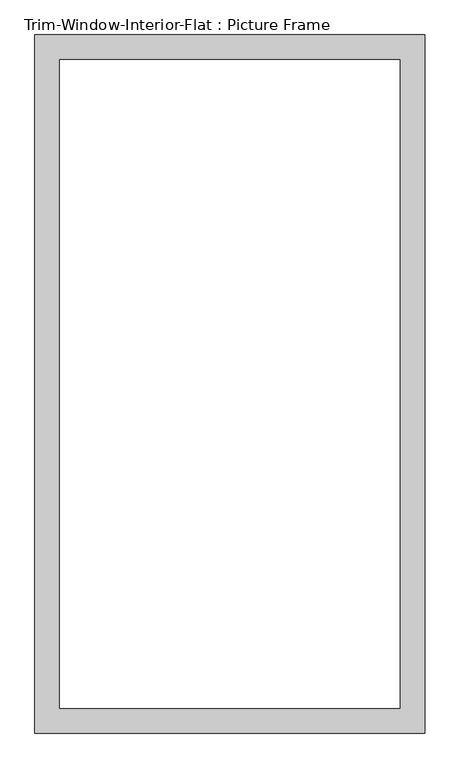
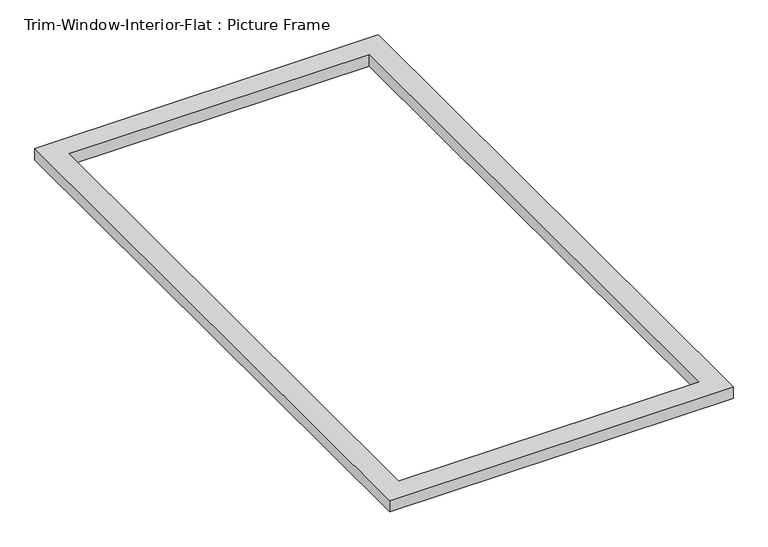
"""IFC4 building model written with IfcOpenShell, lengths in millimetres: proxy geometry, Trim-Window-Interior-Flat : Picture Frame."""

from ifc_helpers import new_model, si_unit, origin, origin_with_axes, place, context, project, spatial, polyline, outline, extrude, source, transform, mapped, element, save


def trim_window_interior_flat_picture_frame_7441b70d(model_context):
    return source(origin(), model_context, "Body", "SweptSolid", [
        extrude(outline(polyline([(450.85, -44.45), (-450.85, -44.45), (-450.85, 1568.45), (450.85, 1568.45), (450.85, -44.45)]), holes=[polyline([(393.7, 12.7), (393.7, 1511.3), (-393.7, 1511.3), (-393.7, 12.7), (393.7, 12.7)])]), origin_with_axes(), (0.0, 0.0, 1.0), 31.75),
    ])


if __name__ == "__main__":
    model = new_model("IFC4")
    model_context = context("Model", 3, world=origin())
    ifc_project = project(units=[si_unit("LENGTHUNIT", "METRE", prefix="MILLI")], contexts=[model_context])
    site = spatial("IfcSite", under=ifc_project)
    building = spatial("IfcBuilding", under=site)
    placement = place(None, origin())
    trim_window_interior_flat_picture_frame_shape = trim_window_interior_flat_picture_frame_7441b70d(model_context)
    element("IfcBuildingElementProxy", 1, Name="Trim-Window-Interior-Flat : Picture Frame", ObjectType="Trim-Window-Interior-Flat : Picture Frame", at=placement, inside=building, context=model_context, shape_type="MappedRepresentation", body=[
        mapped(trim_window_interior_flat_picture_frame_shape, transform((0.0, 0.0, 0.0), x_axis=(1.0, 0.0, 0.0), y_axis=(0.0, 1.0, 0.0), z_axis=(0.0, 0.0, 1.0))),
    ])
    save(model, "model.ifc")

# Revit data of these elements
# Type "Trim-Window-Interior-Flat : Picture Frame"
#   Trim Thickness_Picture Frame = 0' - 1 1/4"
#   Trim Width = 0' - 2 1/4"
#   Trim Thickness_with Sill = 0' - 0 3/4"
#   Sill Thickness = 0' - 1 1/4"
#   Opening Width [instance default] = 2' - 0"
#   Opening Height [instance default] = 3' - 0"
#   Default Elevation = 4' - 0"
#   Sill = no
#   Picture Frame = yes
#   Trim Material [instance default] = none
# Element 1 (IfcBuildingElementProxy, "Trim-Window-Interior-Flat : Picture Frame")
#   Opening Width = 2' - 8"
#   Opening Height = 5' - 0"
#   Trim Material = Wood - Stained
#   Materials on its faces: "Wood - Stained"
# Materials
#   "Wood - Stained": class "Wood", colour RGB 224 178 126, transparency 0, Cost = 0
